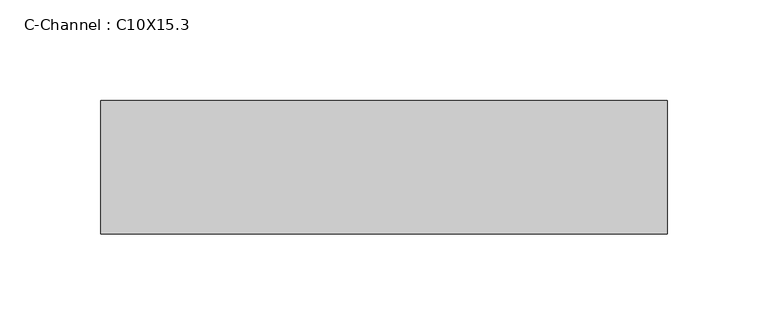
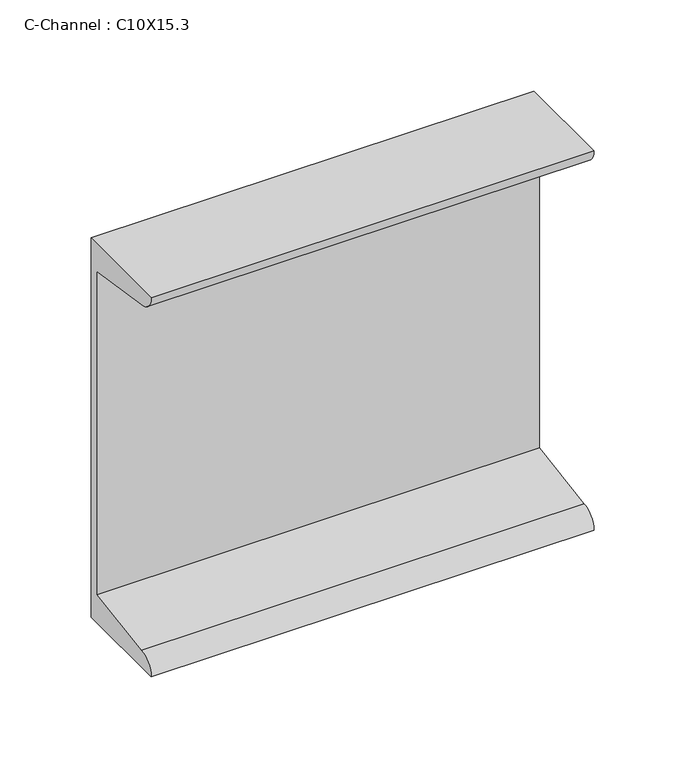
"""IFC4 building model written with IfcOpenShell, lengths in millimetres: beam geometry, C-Channel : C10X15.3."""

from ifc_helpers import new_model, si_unit, point, frame, frame_2d, origin, place, context, project, spatial, polyline, circle_curve, trimmed, segment, composite_curve, outline, extrude, source, transform, mapped, element, save


def c_channel_c10x15_3_20a43f25(model_context):
    return source(origin(), model_context, "Body", "SweptSolid", [
        extrude(outline(composite_curve([segment(polyline([(16.1036, 127.0), (16.1036, -127.0), (-49.9364, -127.0)]), True, "CONTINUOUS"), segment(trimmed(circle_curve(frame_2d((-38.862, -127.0)), 11.0744), [point((-49.9364, -127.0))], [point((-38.862, -115.9256))], False, "CARTESIAN"), True, "CONTINUOUS"), segment(polyline([(-38.862, -115.9256), (10.0076, -108.1854158), (10.0076, 108.1854158), (-38.862, 115.9256)]), True, "CONTINUOUS"), segment(trimmed(circle_curve(frame_2d((-38.862, 127.0)), 11.0744), [point((-38.862, 115.9256))], [point((-49.9364, 127.0))], False, "CARTESIAN"), True, "CONTINUOUS"), segment(polyline([(-49.9364, 127.0), (16.1036, 127.0)]), True, "CONTINUOUS")], self_intersect=False)), frame((-128.27, 0.0, 0.0), z_axis=(1.0, 0.0, 0.0), x_axis=(0.0, 1.0, 0.0)), (0.0, 0.0, 1.0), 280.67),
    ])


if __name__ == "__main__":
    model = new_model("IFC4")
    model_context = context("Model", 3, world=origin())
    ifc_project = project(units=[si_unit("LENGTHUNIT", "METRE", prefix="MILLI")], contexts=[model_context])
    site = spatial("IfcSite", under=ifc_project)
    building = spatial("IfcBuilding", under=site)
    placement = place(None, origin())
    c_channel_c10x15_3_shape = c_channel_c10x15_3_20a43f25(model_context)
    element("IfcBeam", 1, ObjectType="C-Channel : C10X15.3", at=placement, inside=building, context=model_context, shape_type="MappedRepresentation", body=[
        mapped(c_channel_c10x15_3_shape, transform((0.0, 0.0, 0.0), x_axis=(1.0, 0.0, 0.0), y_axis=(0.0, 1.0, 0.0), z_axis=(0.0, 0.0, 1.0))),
    ])
    save(model, "model.ifc")

# Revit data of these elements
# Type "C-Channel : C10X15.3"
#   Assembly Code = "B10"
#   W = 15.3
#   Length [instance default] = 5' - 0"
#   bf = 0' - 2.6"
#   d = 0' - 10"
#   tf = 0' - 0.436"
#   tw = 0' - 0.24"
#   x = 0' - 0.634"
#   A = 0.0311111 SF
#   Structural Material [instance default] = Steel ASTM A36
# Element 1 (IfcBeam, "C-Channel : C10X15.3")
#   Structural Material = Steel ASTM A992
#   Materials on its faces: "Steel ASTM A992"
# Materials
#   "Steel ASTM A36": class "Metal", colour RGB 199 199 199, transparency 0, Description = "Structural steel, ASTM A36 Grade B, mill finish", Cost = 0
#   "Steel ASTM A992": class "Metal", colour RGB 199 199 199, transparency 0, Description = "Structural steel 50ksi", Cost = 0
